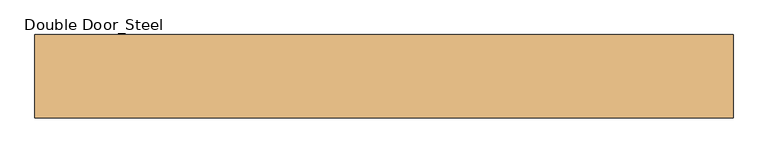
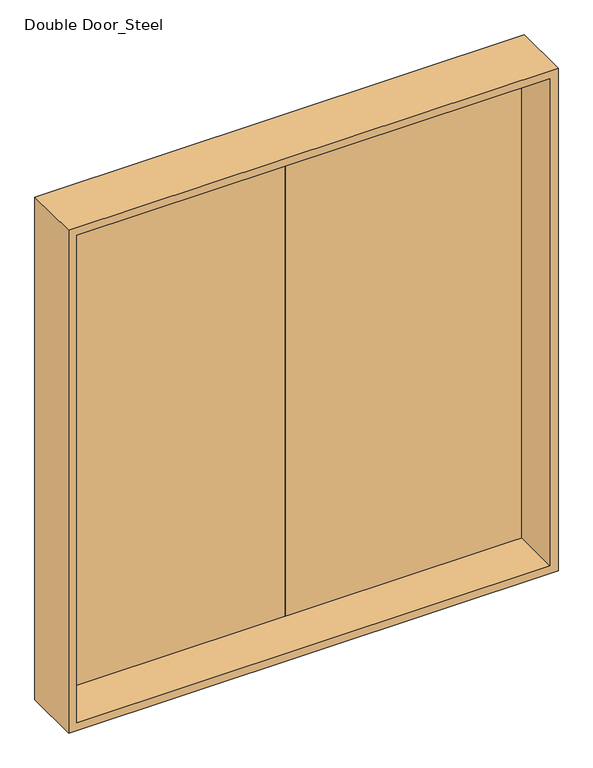
"""IFC4 building model written with IfcOpenShell, lengths in millimetres: door geometry, Double Door_Steel : H_DR_AR_B12_Double Door_Sliding_W2100xH2280_SD3."""

from ifc_helpers import new_model, si_unit, frame, origin, place, context, project, spatial, polyline, outline, extrude, faceted_brep, source, transform, mapped, element, save


def double_door_steel_0cd5a1b8(model_context):
    return source(origin(), model_context, "Body", "SolidModel", [
        extrude(outline(polyline([(1030.0, 85.0), (0.0, 85.0), (0.0, 125.0), (1030.0, 125.0), (1030.0, 85.0)])), frame((0.0, 0.0, 20.0), z_axis=(0.0, 0.0, 1.0), x_axis=(1.0, 0.0, 0.0)), (0.0, 0.0, 1.0), 2240.0),
        extrude(outline(polyline([(0.0, 85.0), (-1030.0, 85.0), (-1030.0, 125.0), (0.0, 125.0), (0.0, 85.0)])), frame((0.0, 0.0, 20.0), z_axis=(0.0, 0.0, 1.0), x_axis=(1.0, 0.0, 0.0)), (0.0, 0.0, 1.0), 2240.0),
        faceted_brep([(1050.0, -125.0, 2280.0), (1050.0, 125.0, 2280.0), (-1050.0, 125.0, 2280.0), (-1050.0, -125.0, 2280.0), (1015.0, 85.0, 2245.0), (1015.0, -125.0, 2245.0), (-1015.0, -125.0, 2245.0), (-1015.0, 85.0, 2245.0), (1030.0, 125.0, 2260.0), (1030.0, 85.0, 2260.0), (-1030.0, 85.0, 2260.0), (-1030.0, 125.0, 2260.0), (-1050.0, 125.0, 0.0), (-1050.0, -125.0, 0.0), (-1015.0, -125.0, 35.0), (-1015.0, 85.0, 35.0), (-1030.0, 85.0, 20.0), (-1030.0, 125.0, 20.0), (1050.0, 125.0, 0.0), (1030.0, 125.0, 20.0), (1050.0, -125.0, 0.0), (1015.0, -125.0, 35.0), (1015.0, 85.0, 35.0), (1030.0, 85.0, 20.0)], [[[0, 1, 2, 3]], [[4, 5, 6, 7]], [[8, 9, 10, 11]], [[3, 2, 12, 13]], [[7, 6, 14, 15]], [[11, 10, 16, 17]], [[18, 12, 2, 1], [8, 11, 17, 19]], [[13, 12, 18, 20]], [[0, 3, 13, 20], [21, 14, 6, 5]], [[15, 14, 21, 22]], [[23, 16, 10, 9], [4, 7, 15, 22]], [[17, 16, 23, 19]], [[20, 18, 1, 0]], [[22, 21, 5, 4]], [[19, 23, 9, 8]]]),
    ])


if __name__ == "__main__":
    model = new_model("IFC4")
    model_context = context("Model", 3, world=origin())
    ifc_project = project(units=[si_unit("LENGTHUNIT", "METRE", prefix="MILLI")], contexts=[model_context])
    site = spatial("IfcSite", under=ifc_project)
    building = spatial("IfcBuilding", under=site)
    placement = place(None, origin())
    double_door_steel_shape = double_door_steel_0cd5a1b8(model_context)
    element("IfcDoor", 1, ObjectType="Double Door_Steel : H_DR_AR_B12_Double Door_Sliding_W2100xH2280_SD3", at=placement, inside=building, context=model_context, shape_type="MappedRepresentation", body=[
        mapped(double_door_steel_shape, transform((0.0, 0.0, 0.0), x_axis=(1.0, 0.0, 0.0), y_axis=(0.0, 1.0, 0.0), z_axis=(0.0, 0.0, 1.0))),
    ])
    save(model, "model.ifc")

# Revit data of these elements
# Type "Double Door_Steel : H_DR_AR_B12_Double Door_Sliding_W2100xH2280_SD3"
#   Type Mark = "445"
#   프레임 = ""
#   철물 = ""
#   유리/마감 = ""
#   위치/개소 = ""
#   부호 = "1/SD"
#   문번호 = "3"
#   문기호 = "SD"
#   Analytic Construction = "<None>"
#   Height = 2280 mm
#   Width = 2100 mm
#   Define Thermal Properties by = 1
#   문 틀 = none
#   문 = none
#   Function = (empty or 0)
#   Assembly Code = ""
#   Wall Closure = (empty or 0)
